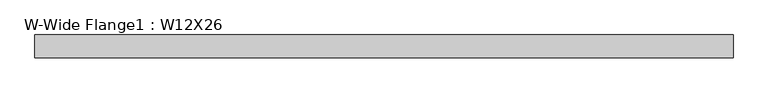
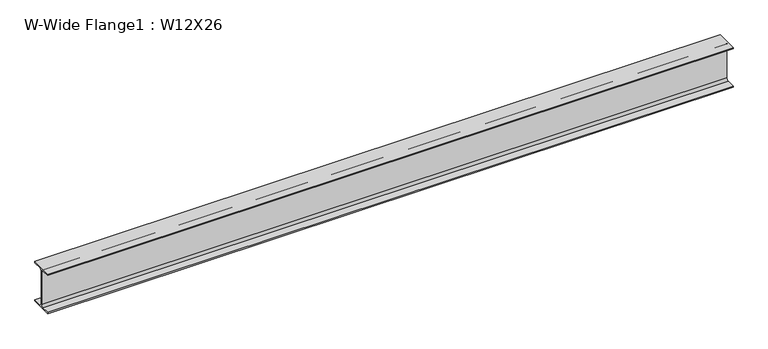
"""IFC4 building model written with IfcOpenShell, lengths in millimetres: beam geometry, W-Wide Flange1 : W12X26."""

from ifc_helpers import new_model, si_unit, point, frame, frame_2d, origin, place, context, project, spatial, polyline, circle_curve, trimmed, segment, composite_curve, outline, extrude, source, transform, mapped, element, save


def w_wide_flange1_w12x26_a5cf21f5(model_context):
    return source(origin(), model_context, "Body", "SweptSolid", [
        extrude(outline(composite_curve([segment(polyline([(82.423, -145.288), (82.423, -154.94), (-82.423, -154.94), (-82.423, -145.288), (-20.2565, -145.288)]), True, "CONTINUOUS"), segment(trimmed(circle_curve(frame_2d((-20.2565, -127.9525)), 17.3355), [point((-20.2565, -145.288))], [point((-2.921, -127.9525))], True, "CARTESIAN"), True, "CONTINUOUS"), segment(polyline([(-2.921, -127.9525), (-2.921, 127.9525)]), True, "CONTINUOUS"), segment(trimmed(circle_curve(frame_2d((-20.2565, 127.9525)), 17.3355), [point((-2.921, 127.9525))], [point((-20.2565, 145.288))], True, "CARTESIAN"), True, "CONTINUOUS"), segment(polyline([(-20.2565, 145.288), (-82.423, 145.288), (-82.423, 154.94), (82.423, 154.94), (82.423, 145.288), (20.2565, 145.288)]), True, "CONTINUOUS"), segment(trimmed(circle_curve(frame_2d((20.2565, 127.9525)), 17.3355), [point((20.2565, 145.288))], [point((2.921, 127.9525))], True, "CARTESIAN"), True, "CONTINUOUS"), segment(polyline([(2.921, 127.9525), (2.921, -127.9525)]), True, "CONTINUOUS"), segment(trimmed(circle_curve(frame_2d((20.2565, -127.9525)), 17.3355), [point((2.921, -127.9525))], [point((20.2565, -145.288))], True, "CARTESIAN"), True, "CONTINUOUS"), segment(polyline([(20.2565, -145.288), (82.423, -145.288)]), True, "CONTINUOUS")], self_intersect=False)), frame((-2535.8079855, 0.0, 0.0), z_axis=(1.0, 0.0, 0.0), x_axis=(0.0, 1.0, 0.0)), (0.0, 0.0, 1.0), 5074.3586468),
    ])


if __name__ == "__main__":
    model = new_model("IFC4")
    model_context = context("Model", 3, world=origin())
    ifc_project = project(units=[si_unit("LENGTHUNIT", "METRE", prefix="MILLI")], contexts=[model_context])
    site = spatial("IfcSite", under=ifc_project)
    building = spatial("IfcBuilding", under=site)
    placement = place(None, origin())
    w_wide_flange1_w12x26_shape = w_wide_flange1_w12x26_a5cf21f5(model_context)
    element("IfcBeam", 1, ObjectType="W-Wide Flange1 : W12X26", at=placement, inside=building, context=model_context, shape_type="MappedRepresentation", body=[
        mapped(w_wide_flange1_w12x26_shape, transform((0.0, 0.0, 0.0), x_axis=(1.0, 0.0, 0.0), y_axis=(0.0, 1.0, 0.0), z_axis=(0.0, 0.0, 1.0))),
    ])
    save(model, "model.ifc")

# Revit data of these elements
# Type "W-Wide Flange1 : W12X26"
#   Assembly Code = "B10"
#   W = 26
#   Start Extension Calculation [instance default] = 10' - 0"
#   Start Extension [instance default] = -0' - 0 1/2"
#   End Extension Calculation [instance default] = 10' - 0"
#   End Extension [instance default] = -0' - 0 1/2"
#   Length [instance default] = 5' - 0"
#   bf = 0' - 6.49"
#   d = 1' - 0.2"
#   k = 0' - 1 1/16"
#   k2 = 0' - 0.6825"
#   tf = 0' - 0.38"
#   tw = 0' - 0.23"
#   A = 0.053125 SF
#   Structural Material [instance default] = Metal - Steel - ASTM A992
# Element 1 (IfcBeam, "W-Wide Flange1 : W12X26")
#   Materials on its faces: "Metal - Steel - ASTM A992"
# Materials
#   "Metal - Steel - ASTM A992": class "Metal", colour RGB 199 199 199, transparency 0
